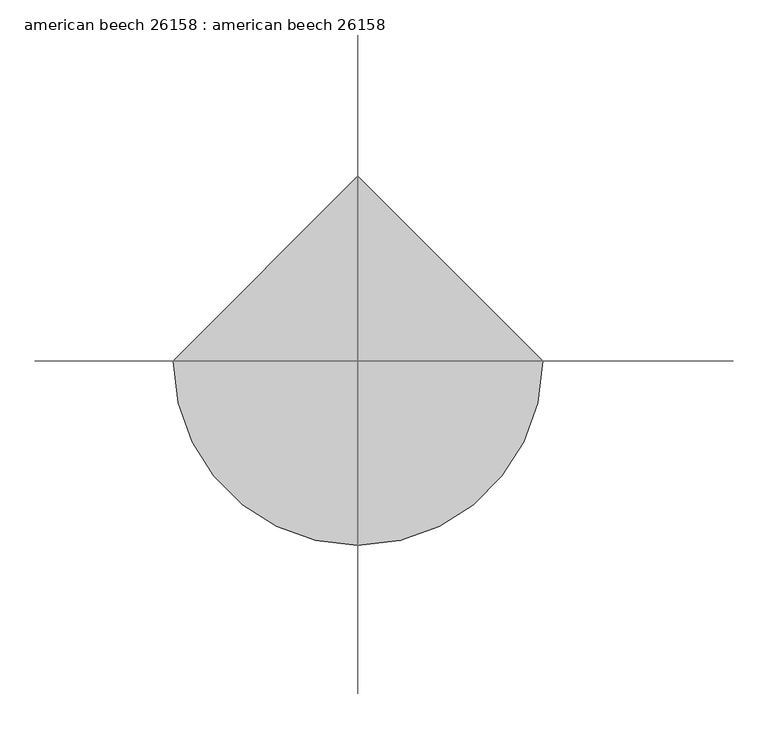
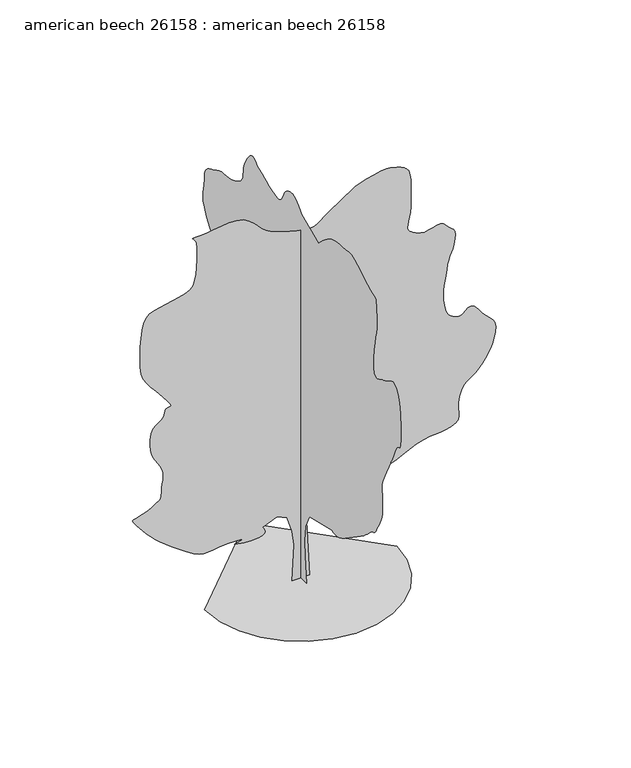
"""IFC4 building model written with IfcOpenShell, lengths in millimetres: proxy geometry, american beech 26158 : american beech 26158."""

import ifcopenshell
import ifcopenshell.guid

model = None  # the IFC model being written
_history = None  # IfcOwnerHistory: only IFC2X3 demands one
_inside = {}  # id of a spatial element -> (the spatial element, [elements in it])
_under = {}  # id of a project, library or spatial element -> (it, [spatial elements below it])
_declared = {}  # id of a project -> (the project, [libraries it declares])
_typed = {}  # id of a type object -> (the type object, [elements of that type])
_made_of = {}  # id of a material, layer set ... -> (it, [elements and type objects made of it])


def new_model(schema):
    """Start an empty IFC model of exactly this schema.

    Asked for "IFC4X3", IfcOpenShell would pick the latest addendum, in which some entities
    have other attributes; the version numbers below select the first issue.
    IFC2X3 requires an IfcOwnerHistory on every rooted entity: one is made here for all.
    """
    global model, _history
    if schema == "IFC4X3":
        model = ifcopenshell.file(schema_version=(4, 3, 0, 0))
    else:
        model = ifcopenshell.file(schema=schema)
    _inside.clear()
    _under.clear()
    _declared.clear()
    _typed.clear()
    _made_of.clear()
    _history = None
    if model.schema == "IFC2X3":
        org = make("IfcOrganization", Name="unknown")
        user = make(
            "IfcPersonAndOrganization",
            ThePerson=make("IfcPerson", FamilyName="unknown"),
            TheOrganization=org,
        )
        app = make(
            "IfcApplication",
            ApplicationDeveloper=org,
            Version="unknown",
            ApplicationFullName="unknown",
            ApplicationIdentifier="unknown",
        )
        _history = make(
            "IfcOwnerHistory",
            OwningUser=user,
            OwningApplication=app,
            ChangeAction="ADDED",
            CreationDate=0,
        )
    return model


def make(cls, **values):
    """One entity of the class cls with the attributes given. An attribute that is None is left unset."""
    return model.create_entity(
        cls, **{name: value for name, value in values.items() if value is not None}
    )


def rooted(cls, **values):
    """An entity with a GlobalId (a new one), such as an element, a storey or a relation."""
    return make(cls, GlobalId=ifcopenshell.guid.new(), OwnerHistory=_history, **values)


def si_unit(unit_type, name, prefix=None):
    """IfcSIUnit, for example si_unit("LENGTHUNIT", "METRE", prefix="MILLI")."""
    return make("IfcSIUnit", UnitType=unit_type, Prefix=prefix, Name=name)


def assignment(units):
    """IfcUnitAssignment: the units of a project."""
    return None if units is None else make("IfcUnitAssignment", Units=units)


def point(xyz):
    """IfcCartesianPoint."""
    return None if xyz is None else make("IfcCartesianPoint", Coordinates=xyz)


def direction(xyz):
    """IfcDirection."""
    return None if xyz is None else make("IfcDirection", DirectionRatios=xyz)


def frame(location, z_axis=None, x_axis=None):
    """IfcAxis2Placement3D, a coordinate frame: its origin and axes. An axis left out is left unset."""
    return make(
        "IfcAxis2Placement3D",
        Location=point(location),
        Axis=direction(z_axis),
        RefDirection=direction(x_axis),
    )


def origin():
    """The frame at (0, 0, 0) with its axes left unset."""
    return frame((0.0, 0.0, 0.0))


def place(relative_to, where):
    """IfcLocalPlacement: puts the frame where relative to a parent placement (None: the world)."""
    return make(
        "IfcLocalPlacement", PlacementRelTo=relative_to, RelativePlacement=where
    )


def context(
    kind, dimensions, precision=None, world=None, true_north=None, identifier=None
):
    """IfcGeometricRepresentationContext, for example the 3D "Model" context."""
    return make(
        "IfcGeometricRepresentationContext",
        ContextIdentifier=identifier,
        ContextType=kind,
        CoordinateSpaceDimension=dimensions,
        Precision=precision,
        WorldCoordinateSystem=world,
        TrueNorth=true_north,
    )


def project(units=None, contexts=None):
    """IfcProject with its units and contexts."""
    return rooted(
        "IfcProject",
        Name="project",
        RepresentationContexts=contexts,
        UnitsInContext=assignment(units),
    )


def spatial(cls, under=None, at=None, **own):
    """A site, building, storey or space (cls), placed at a placement, below another one or the project."""
    s = rooted(cls, ObjectPlacement=at, **own)
    if under is not None:
        _under.setdefault(under.id(), (under, []))[1].append(s)
    return s


def point_list(points):
    """IfcCartesianPointList2D or 3D."""
    cls = (
        "IfcCartesianPointList2D" if len(points[0]) == 2 else "IfcCartesianPointList3D"
    )
    return make(cls, CoordList=points)


def triangles(points, corners, closed=None, point_numbers=None):
    """IfcTriangulatedFaceSet: each triangle names its three corners, points numbered from 1."""
    return make(
        "IfcTriangulatedFaceSet",
        Coordinates=point_list(points),
        Closed=closed,
        CoordIndex=corners,
        PnIndex=point_numbers,
    )


def shape(context_of_items, identifier, shape_type, items):
    """IfcShapeRepresentation: the items that make up one representation, for example the "Body"."""
    return make(
        "IfcShapeRepresentation",
        ContextOfItems=context_of_items,
        RepresentationIdentifier=identifier,
        RepresentationType=shape_type,
        Items=items,
    )


def source(mapping_origin, context_of_items, identifier, shape_type, items):
    """IfcRepresentationMap: a shape defined once, which mapped items show again and again."""
    return make(
        "IfcRepresentationMap",
        MappingOrigin=mapping_origin,
        MappedRepresentation=shape(context_of_items, identifier, shape_type, items),
    )


def transform(
    local_origin,
    x_axis=None,
    y_axis=None,
    z_axis=None,
    scale=None,
    scale2=None,
    scale3=None,
    uniform=True,
):
    """IfcCartesianTransformationOperator3D, or its non-uniform kind. x_axis, y_axis, z_axis: its Axis1, 2, 3."""
    if uniform:
        return make(
            "IfcCartesianTransformationOperator3D",
            Axis1=direction(x_axis),
            Axis2=direction(y_axis),
            LocalOrigin=point(local_origin),
            Scale=scale,
            Axis3=direction(z_axis),
        )
    return make(
        "IfcCartesianTransformationOperator3DnonUniform",
        Axis1=direction(x_axis),
        Axis2=direction(y_axis),
        LocalOrigin=point(local_origin),
        Scale=scale,
        Axis3=direction(z_axis),
        Scale2=scale2,
        Scale3=scale3,
    )


def mapped(mapping_source, mapping_target):
    """IfcMappedItem: shows the shape of a source again, moved by a transform."""
    return make(
        "IfcMappedItem", MappingSource=mapping_source, MappingTarget=mapping_target
    )


def made_of(thing, what):
    """Note that an element or type object is made of a material, layer set ...; save() writes the relation."""
    if what is not None:
        _made_of.setdefault(what.id(), (what, []))[1].append(thing)
    return thing


def element(
    cls,
    number,
    at=None,
    inside=None,
    cuts=None,
    type_object=None,
    material=None,
    context=None,
    identifier="Body",
    shape_type=None,
    held_by="IfcProductDefinitionShape",
    body=None,
    shapes=None,
    **own,
):
    """One element of the class cls, such as IfcWall. Its Tag is "e" and its number.

    at: its placement. inside: the storey or other place that contains it. cuts: it is an
    opening in that element (IfcRelVoidsElement). A single representation is given by context,
    identifier, shape_type and body (its items); several are given by shapes. held_by: the class
    of the entity that holds the representations. save() writes the other relations.
    """
    e = rooted(cls, Tag="e%d" % number, ObjectPlacement=at, **own)
    if body is not None:
        shapes = [shape(context, identifier, shape_type, body)]
    if shapes is not None:
        e.Representation = make(held_by, Representations=shapes)
    if inside is not None:
        _inside.setdefault(inside.id(), (inside, []))[1].append(e)
    if cuts is not None:
        rooted(
            "IfcRelVoidsElement", RelatingBuildingElement=cuts, RelatedOpeningElement=e
        )
    if type_object is not None:
        _typed.setdefault(type_object.id(), (type_object, []))[1].append(e)
    return made_of(e, material)


def aggregate(whole, parts):
    """IfcRelAggregates: a whole, such as a stair, and the parts it consists of."""
    return rooted("IfcRelAggregates", RelatingObject=whole, RelatedObjects=parts)


def save(model, path):
    """Write the relations noted so far, then the file.

    IfcRelAggregates (storeys below a building ...), IfcRelContainedInSpatialStructure (elements
    in a storey), IfcRelDefinesByType, IfcRelAssociatesMaterial and IfcRelDeclares: one each for
    every whole, place, type object, material and project.
    """
    for whole, parts in _under.values():
        aggregate(whole, parts)
    for where, things in _inside.values():
        rooted(
            "IfcRelContainedInSpatialStructure",
            RelatedElements=things,
            RelatingStructure=where,
        )
    for kind, things in _typed.values():
        rooted("IfcRelDefinesByType", RelatedObjects=things, RelatingType=kind)
    for what, things in _made_of.values():
        rooted("IfcRelAssociatesMaterial", RelatedObjects=things, RelatingMaterial=what)
    for by, libraries in _declared.values():
        rooted("IfcRelDeclares", RelatingContext=by, RelatedDefinitions=libraries)
    model.write(path)


def american_beech_26158_american_beech_26158_b3c041c8(model_context):
    return source(origin(), model_context, "Body", "Tessellation", [
        triangles([(0.0009889, 136.856581, 0.0), (0.0009889, -149.8547884, 0.0), (0.0009889, -111.6264895, 420.510052), (0.0009889, -102.0697236, 659.4353302), (0.0009889, -121.1832463, 898.3606447), (0.0009889, -235.8678885, 1118.172373), (0.0009889, -818.8458761, 1261.5275036), (0.0009889, -849.9431059, 1249.7139805), (0.0009889, -883.2933231, 1240.7427258), (0.0009889, -921.1596891, 1237.4533916), (0.0009889, -965.7976622, 1242.6934788), (0.0009889, -1019.4603024, 1259.3000233), (0.0009889, -1084.4081549, 1290.1152935), (0.0009889, -1162.8992941, 1337.984174), (0.0009889, -1478.2811337, 1557.7959023), (0.0009889, -1522.8632961, 1589.1420994), (0.0009889, -1566.942437, 1618.9819931), (0.0009889, -1611.1893002, 1649.3249084), (0.0009889, -1656.2718681, 1682.1772636), (0.0009889, -1702.8579781, 1719.5406807), (0.0009889, -1751.6183739, 1763.4243393), (0.0009889, -1803.2210381, 1815.834803), (0.0009889, -1847.9404015, 1858.0191467), (0.0009889, -1878.9512993, 1877.1351311), (0.0009889, -1901.2702858, 1884.0440117), (0.0009889, -1919.9112991, 1889.616782), (0.0009889, -1939.8884228, 1904.7196392), (0.0009889, -1966.2180656, 1940.2161644), (0.0009889, -2003.916782, 2006.9774963), (0.0009889, -2044.9607883, 2083.2080177), (0.0009889, -2078.313549, 2145.2324295), (0.0009889, -2104.4754696, 2201.0692829), (0.0009889, -2123.9521877, 2258.7475937), (0.0009889, -2137.244109, 2326.2862038), (0.0009889, -2144.8488773, 2411.7141289), (0.0009889, -2147.2746014, 2523.0550072), (0.0009889, -2142.5373905, 2624.8889076), (0.0009889, -2132.7863869, 2688.2873634), (0.0009889, -2124.7040314, 2730.9338882), (0.0009889, -2124.9835201, 2770.583503), (0.0009889, -2140.3072941, 2824.9394875), (0.0009889, -2177.3659332, 2911.7568626), (0.0009889, -2242.84464, 3048.6883301), (0.0009889, -2308.7119858, 3181.9621719), (0.0009889, -2348.5011269, 3259.3812836), (0.0009889, -2371.2366577, 3301.215358), (0.0009889, -2385.9484051, 3327.6567673), (0.0009889, -2401.6632889, 3358.9496246), (0.0009889, -2427.4088104, 3415.3121727), (0.0009889, -2472.2118896, 3516.9885246), (0.0009889, -2522.8114174, 3609.6476944), (0.0009889, -2561.0332123, 3645.1568642), (0.0009889, -2588.5669968, 3652.9040657), (0.0009889, -2607.0580193, 3662.3273277), (0.0009889, -2618.2087921, 3702.8402618), (0.0009889, -2623.669796, 3803.856189), (0.0009889, -2625.117382, 3994.8390083), (0.0009889, -2615.3639076, 4210.713913), (0.0009889, -2589.2271309, 4371.4450905), (0.0009889, -2551.406765, 4483.8402649), (0.0009889, -2506.5400269, 4554.7824463), (0.0009889, -2459.3391289, 4591.1043571), (0.0009889, -2414.4802391, 4599.6895889), (0.0009889, -2376.641851, 4587.3705734), (0.0009889, -2343.8477772, 4566.9491455), (0.0009889, -2310.8862717, 4546.8576393), (0.0009889, -2277.5893215, 4527.4521378), (0.0009889, -2243.7921112, 4509.0116936), (0.0009889, -2209.3243023, 4491.9426773), (0.0009889, -2174.0232594, 4476.5250137), (0.0009889, -2137.7164639, 4463.1392029), (0.0009889, -2096.4236355, 4443.6572525), (0.0009889, -2049.6139927, 4418.4858238), (0.0009889, -2002.3013283, 4400.6805153), (0.0009889, -1959.504958, 4403.2713455), (0.0009889, -1926.2359131, 4439.313913), (0.0009889, -1907.5110386, 4521.8132378), (0.0009889, -1908.3467434, 4663.8246277), (0.0009889, -1923.6450829, 4819.4253044), (0.0009889, -1942.954224, 4940.7356323), (0.0009889, -1963.266647, 5037.9669067), (0.0009889, -1981.572361, 5121.3298416), (0.0009889, -1994.8642822, 5201.0354416), (0.0009889, -2000.1296585, 5287.2429703), (0.0009889, -1994.3614059, 5390.1634323), (0.0009889, -1986.3653824, 5488.9190323), (0.0009889, -1983.048143, 5559.911792), (0.0009889, -1978.5625156, 5609.3407516), (0.0009889, -1967.0562412, 5643.3764648), (0.0009889, -1942.6748806, 5668.2429703), (0.0009889, -1899.5709709, 5690.0869858), (0.0009889, -1831.8926891, 5715.1063889), (0.0009889, -1748.4408062, 5751.9616974), (0.0009889, -1662.820015, 5800.5261749), (0.0009889, -1576.3582867, 5853.7903656), (0.0009889, -1490.4020508, 5904.6919098), (0.0009889, -1406.2848015, 5946.2207703), (0.0009889, -1325.3426491, 5971.3924896), (0.0009889, -1248.913884, 5973.1447083), (0.0009889, -1174.2403896, 5963.3406555), (0.0009889, -1098.5636135, 5956.711409), (0.0009889, -1023.222064, 5950.5641098), (0.0009889, -949.5518515, 5942.2588028), (0.0009889, -878.8914843, 5929.1264648), (0.0009889, -812.5771454, 5908.4509827), (0.0009889, -751.9472706, 5877.5644958), (0.0009889, -697.9494038, 5841.2678741), (0.0009889, -649.9687569, 5805.9618896), (0.0009889, -607.0045916, 5771.4942261), (0.0009889, -568.0511189, 5737.7119858), (0.0009889, -532.1075644, 5704.4128555), (0.0009889, -498.1706097, 5671.4433563), (0.0009889, -465.2369368, 5638.6523346), (0.0009889, -16.056217, 5829.7871796), (0.0009889, 22.8405617, 5872.4339951), (0.0009889, 61.6537222, 5913.023378), (0.0009889, 100.2998553, 5949.3961578), (0.0009889, 138.6950317, 5979.5204819), (0.0009889, 176.7559443, 6001.2883392), (0.0009889, 214.3990318, 6012.5911377), (0.0009889, 251.5404602, 6011.3720261), (0.0009889, 287.2056524, 6002.4312927), (0.0009889, 320.3628219, 5991.305809), (0.0009889, 350.8454089, 5977.0055191), (0.0009889, 378.4856913, 5958.5397858), (0.0009889, 403.1160919, 5934.892392), (0.0009889, 424.5689612, 5905.047702), (0.0009889, 442.6817001, 5868.0144974), (0.0009889, 459.9562634, 5826.9425858), (0.0009889, 480.2407084, 5787.547316), (0.0009889, 505.3740581, 5752.6727005), (0.0009889, 537.1926464, 5725.138916), (0.0009889, 577.5380399, 5707.7911377), (0.0009889, 628.2491524, 5703.5239563), (0.0009889, 691.1650068, 5715.1063889), (0.0009889, 759.6790661, 5736.9754028), (0.0009889, 826.1890326, 5761.3593796), (0.0009889, 891.0251186, 5787.8263687), (0.0009889, 954.5251671, 5815.9694183), (0.0009889, 1017.0218611, 5845.3577408), (0.0009889, 1078.8506453, 5875.5832214), (0.0009889, 1140.3440575, 5906.2412338), (0.0009889, 1169.0715191, 5932.3524307), (0.0009889, 1198.1316639, 5955.3649796), (0.0009889, 1227.8624073, 5972.2052307), (0.0009889, 1258.5938164, 5979.7489563), (0.0009889, 1290.6664227, 5974.9230881), (0.0009889, 1324.4078224, 5954.6539764), (0.0009889, 1360.1557858, 5915.7918137), (0.0009889, 1395.1799561, 5868.217392), (0.0009889, 1426.1908539, 5822.9544571), (0.0009889, 1452.6880737, 5778.8856354), (0.0009889, 1474.1715008, 5734.7912338), (0.0009889, 1490.1379681, 5689.5538788), (0.0009889, 1500.0845993, 5641.9538773), (0.0009889, 1503.510989, 5590.8494385), (0.0009889, 1507.2168674, 5539.3380478), (0.0009889, 1519.1142517, 5491.1793594), (0.0009889, 1540.3740005, 5446.1704788), (0.0009889, 1572.1672634, 5404.1846695), (0.0009889, 1615.6596668, 5365.0428726), (0.0009889, 1672.0274471, 5328.5689362), (0.0009889, 1742.4363762, 5294.5832199), (0.0009889, 1817.5288857, 5269.1836075), (0.0009889, 1887.9378147, 5255.1373718), (0.0009889, 1954.8363476, 5247.4407486), (0.0009889, 2019.3956337, 5241.0911362), (0.0009889, 2082.7839157, 5231.0580276), (0.0009889, 2146.1721977, 5212.3382401), (0.0009889, 2210.7313385, 5179.9024292), (0.0009889, 2276.3498623, 5145.3580261), (0.0009889, 2340.1267834, 5118.8404587), (0.0009889, 2399.0573433, 5093.1356323), (0.0009889, 2450.1315514, 5061.106192), (0.0009889, 2490.3372368, 5015.5136261), (0.0009889, 2516.667025, 4949.193837), (0.0009889, 2526.1132507, 4854.9597633), (0.0009889, 2532.46577, 4758.008123), (0.0009889, 2546.5044479, 4681.9348595), (0.0009889, 2560.7285797, 4617.2411339), (0.0009889, 2567.5865913, 4554.3760757), (0.0009889, 2559.5600464, 4483.8402649), (0.0009889, 2529.1232414, 4396.0578323), (0.0009889, 2468.7702393, 4281.5543564), (0.0009889, 2394.0992157, 4166.6192207), (0.0009889, 2326.6139454, 4078.2525215), (0.0009889, 2267.6553349, 4007.9707649), (0.0009889, 2218.5596397, 3947.1884285), (0.0009889, 2180.6679119, 3887.4223091), (0.0009889, 2155.3111748, 3820.1377533), (0.0009889, 2143.8328056, 3736.8001076), (0.0009889, 2149.4334812, 3646.0204742), (0.0009889, 2171.0820145, 3561.7686401), (0.0009889, 2203.7667927, 3483.5112076), (0.0009889, 2242.4687908, 3410.790937), (0.0009889, 2282.1714546, 3343.1000107), (0.0009889, 2317.8662235, 3279.9047401), (0.0009889, 2344.5311657, 3220.7225967), (0.0009889, 2370.3577869, 3180.6921913), (0.0009889, 2402.5396889, 3164.8934464), (0.0009889, 2434.5538685, 3157.7813805), (0.0009889, 2459.8827003, 3143.8113029), (0.0009889, 2472.0037628, 3107.4638123), (0.0009889, 2464.3963783, 3033.1433487), (0.0009889, 2430.5432121, 2905.3305107), (0.0009889, 2383.9011463, 2761.3378464), (0.0009889, 2340.6017544, 2643.9136185), (0.0009889, 2298.1379219, 2545.7425758), (0.0009889, 2254.0028252, 2459.415287), (0.0009889, 2205.6894951, 2377.6095245), (0.0009889, 2150.6857304, 2292.9614937), (0.0009889, 2086.4897942, 2198.1177189), (0.0009889, 2022.098085, 2102.5196297), (0.0009889, 1968.0723129, 2019.6267242), (0.0009889, 1924.2446102, 1948.102747), (0.0009889, 1890.4447838, 1886.6067913), (0.0009889, 1866.5103436, 1833.8078339), (0.0009889, 1852.2735672, 1788.3620613), (0.0009889, 1847.564407, 1748.9361248), (0.0009889, 1851.5776794, 1721.8800728), (0.0009889, 1860.940044, 1709.2029396), (0.0009889, 1871.6386642, 1703.0459026), (0.0009889, 1879.6624477, 1695.5504299), (0.0009889, 1881.0010288, 1678.8600243), (0.0009889, 1871.6386642, 1645.1186245), (0.0009889, 1847.564407, 1586.4675533), (0.0009889, 1827.5314728, 1524.5828133), (0.0009889, 1825.3850922, 1482.2587978), (0.0009889, 1829.7590984, 1453.3104195), (0.0009889, 1829.2865982, 1431.547649), (0.0009889, 1812.5961926, 1410.7907764), (0.0009889, 1768.3214241, 1384.8497726), (0.0009889, 1685.0958355, 1347.5421661), (0.0009889, 1594.399918, 1309.4244347), (0.0009889, 1528.281134, 1282.5080544), (0.0009889, 1476.2059696, 1262.7823689), (0.0009889, 1427.6412014, 1246.2316349), (0.0009889, 1372.05317, 1228.8453415), (0.0009889, 1298.9138844, 1206.6102161), (0.0009889, 1197.6871416, 1175.5154572), (0.0009889, 1096.069289, 1145.7009253), (0.0009889, 1022.5387482, 1127.7557997), (0.0009889, 967.7331545, 1118.3400227), (0.0009889, 922.2874546, 1114.10329), (0.0009889, 876.8442255, 1111.7080873), (0.0009889, 822.0360884, 1107.806654), (0.0009889, 748.5055475, 1099.0588594), (0.0009889, 662.4935011, 1085.0990284), (0.0009889, 576.4788749, 1068.1292793), (0.0009889, 490.4667558, 1048.6551046), (0.0009889, 404.4521296, 1027.1717503), (0.0009889, 318.4400468, 1004.1847086), (0.0009889, 232.4266923, 980.1943851), (0.0009889, 146.4133378, 955.7037289), (136.1842383, 0.0003154, 0.014068), (-131.4120823, 0.0003154, 0.014068), (-102.7410489, 0.0002819, 563.8778998), (-131.4120823, 0.0002692, 793.2477293), (-207.8684348, 0.0002549, 1032.1729712), (-360.7819027, 0.0002501, 1108.6296415), (-580.5936673, 0.0002549, 1013.0594576), (-562.704425, 0.0002564, 988.5662579), (-548.0765751, 0.000258, 964.5784779), (-539.9688578, 0.0002596, 941.5914362), (-541.6401947, 0.0002612, 920.1080818), (-556.3518694, 0.0002628, 900.6313637), (-587.3627672, 0.0002628, 883.6641581), (-637.9342443, 0.0002644, 869.704327), (-697.421093, 0.0002644, 860.4815615), (-753.4001616, 0.0002644, 856.775683), (-806.4506298, 0.0002644, 857.667271), (-857.1617786, 0.0002644, 862.2366869), (-906.117802, 0.0002644, 869.5645826), (-953.9028214, 0.0002628, 878.731465), (-1001.1011759, 0.0002628, 888.8178406), (-953.2881786, 0.0002628, 900.9945683), (-913.501581, 0.0002612, 912.5008427), (-889.7601522, 0.0002612, 922.6710068), (-890.0954515, 0.0002596, 930.8345346), (-922.5287189, 0.0002596, 936.3235165), (-995.0838833, 0.0002596, 938.4698244), (-1115.7848007, 0.0002596, 936.6028599), (-1242.9524746, 0.0002612, 927.8271601), (-1337.3542706, 0.0002612, 914.3677345), (-1410.6891838, 0.0002612, 903.2500992), (-1474.6617325, 0.0002612, 901.4949738), (-1540.9759987, 0.0002612, 916.12286), (-1621.3340298, 0.0002596, 954.1568756), (-1727.4351116, 0.0002549, 1022.614979), (-1845.0726986, 0.0002501, 1105.8432564), (-1952.34711, 0.0002453, 1184.0549795), (-2049.4209812, 0.0002405, 1258.0858532), (-2136.46436, 0.0002373, 1328.7765965), (-2213.6472942, 0.0002326, 1396.9554291), (-2281.1300938, 0.0002278, 1463.4653229), (-2339.0852772, 0.0002246, 1529.1396572), (-2391.8031349, 0.0002214, 1592.6651402), (-2441.3431343, 0.0002166, 1651.1791557), (-2484.5309052, 0.0002134, 1703.170459), (-2518.1884438, 0.0002118, 1747.1378334), (-2539.1409439, 0.0002103, 1781.577737), (-2544.218541, 0.0002087, 1804.9838665), (-2530.2254997, 0.0002071, 1815.8500637), (-2498.742247, 0.0002071, 1822.7308937), (-2456.2227493, 0.0002071, 1834.628278), (-2406.8475655, 0.0002055, 1850.7065117), (-2354.8003063, 0.0002039, 1870.1272739), (-2304.2568798, 0.0002023, 1892.0551506), (-2259.3978447, 0.0002023, 1915.6542915), (-2224.401725, 0.0002007, 1940.091608), (-2196.9849392, 0.0001991, 1958.6464348), (-2172.4078056, 0.0001991, 1969.1798035), (-2151.1759621, 0.0001975, 1977.7066086), (-2133.7896687, 0.0001975, 1990.2439247), (-2120.7518017, 0.0001959, 2012.8144947), (-2112.5602959, 0.0001927, 2051.4326317), (-2109.7180275, 0.0001895, 2112.118317), (-2105.7607109, 0.0001864, 2181.0514641), (-2096.7894562, 0.0001816, 2242.2935108), (-2087.1476028, 0.0001784, 2298.6891964), (-2081.1861935, 0.0001752, 2353.0781731), (-2083.2487129, 0.000172, 2408.3028545), (-2097.6809715, 0.0001688, 2467.2028931), (-2128.8315411, 0.0001641, 2532.6259346), (-2168.3971493, 0.0001609, 2596.7202782), (-2204.2849297, 0.0001577, 2653.2860115), (-2235.1560104, 0.0001545, 2707.6675758), (-2259.6771881, 0.0001513, 2765.2239464), (-2276.5047947, 0.0001465, 2831.3149704), (-2284.3076614, 0.0001418, 2911.2740433), (-2281.7447365, 0.000137, 3010.4865921), (-2264.5514545, 0.0001306, 3102.7902603), (-2233.1494469, 0.0001274, 3164.9948936), (-2193.2231049, 0.0001242, 3206.8286774), (-2150.4520237, 0.0001226, 3237.9439293), (-2110.525827, 0.0001211, 3268.0682533), (-2079.123674, 0.0001179, 3306.8795471), (-2061.9330082, 0.0001147, 3364.0804161), (-2043.9599773, 0.0001131, 3413.0262657), (-2014.1200836, 0.0001115, 3431.3396828), (-1983.9422745, 0.0001115, 3435.3019409), (-1964.9684326, 0.0001099, 3441.0931572), (-1968.7301216, 0.0001099, 3464.9437363), (-2006.7641373, 0.0001051, 3523.0843735), (-2090.6020432, 9.88e-05, 3631.6948952), (-2191.4121689, 9.24e-05, 3753.7165169), (-2273.3296978, 8.6e-05, 3849.6778107), (-2337.3582024, 8.12e-05, 3932.1009773), (-2384.5031445, 7.65e-05, 4013.5079269), (-2415.7654804, 7.17e-05, 4106.47202), (-2432.1484921, 6.37e-05, 4223.4898773), (-2434.6554611, 5.42e-05, 4377.1345688), (-2429.5297565, 4.46e-05, 4541.5998207), (-2420.5585018, 3.66e-05, 4683.0016548), (-2405.0643894, 3.03e-05, 4801.6705742), (-2380.3781055, 2.39e-05, 4897.9365005), (-2343.822488, 1.91e-05, 4972.1558075), (-2292.720084, 1.59e-05, 5024.6066757), (-2224.401725, 1.43e-05, 5055.6710587), (-2138.4149677, 1.27e-05, 5074.7972168), (-2040.8941761, 1.27e-05, 5092.7292618), (-1939.0274288, 1.11e-05, 5111.8554199), (-1840.0028046, 9.6e-06, 5134.487178), (-1751.0088181, 8e-06, 5162.9604401), (-1679.2334026, 6.4e-06, 5199.612854), (-1631.8649277, 3.2e-06, 5246.8314835), (-1604.1128426, -1.6e-06, 5316.4272354), (-1585.3905842, -6.4e-06, 5411.6010773), (-1574.1890877, -1.27e-05, 5521.6594757), (-1569.0075726, -2.07e-05, 5635.9088974), (-1568.336974, -2.71e-05, 5743.6302292), (-1570.6788368, -3.19e-05, 5834.1305191), (-1574.524387, -3.5e-05, 5896.690654), (-1585.918895, -3.82e-05, 5936.1626633), (-1606.0102558, -3.98e-05, 5965.4230865), (-1625.9315689, -4.14e-05, 5985.9718323), (-1636.825526, -4.14e-05, 5999.3576431), (-1629.8329296, -4.3e-05, 6007.0286865), (-1596.0890591, -4.3e-05, 6010.559285), (-1526.7393677, -4.3e-05, 6011.3976059), (-1428.7715103, -4.3e-05, 6017.8233765), (-1318.7690678, -4.46e-05, 6032.4538788), (-1202.2439129, -4.46e-05, 6048.2529144), (-1084.7180197, -4.46e-05, 6058.184285), (-971.7057318, -4.46e-05, 6055.263533), (-868.7238636, -4.46e-05, 6032.4538788), (-781.2893749, -4.14e-05, 5982.7208679), (-714.8937183, -3.66e-05, 5922.6245361), (-665.5465851, -3.34e-05, 5871.6974121), (-624.5610781, -3.19e-05, 5827.4756927), (-583.2403444, -2.87e-05, 5787.445578), (-532.8924365, -2.71e-05, 5749.0915237), (-464.8228995, -2.39e-05, 5709.8735687), (-370.3373878, -2.23e-05, 5667.3284912), (-260.8632923, -1.91e-05, 5627.3745346), (-155.7366604, -1.75e-05, 5596.9449966), (-58.1322665, -1.59e-05, 5575.0504028), (28.7726351, -1.59e-05, 5560.6739548), (101.8020074, -1.59e-05, 5552.8255966), (157.7788323, -1.43e-05, 5550.4629501), (193.5270681, -1.59e-05, 5552.6477005), (219.2725352, -1.59e-05, 5560.6233765), (247.3583572, -1.59e-05, 5575.4311935), (277.7847885, -1.75e-05, 5595.7770447), (310.5508118, -1.91e-05, 5620.2877579), (345.6587342, -2.07e-05, 5647.6692261), (383.1059761, -2.23e-05, 5676.5232788), (422.8950809, -2.39e-05, 5705.555809), (805.1781057, -3.98e-05, 5963.5947098), (830.3647951, -3.98e-05, 5972.992392), (896.679134, -4.14e-05, 5996.5892075), (990.2426817, -4.3e-05, 6027.5518524), (1097.1817938, -4.62e-05, 6058.9970261), (1203.6180296, -4.62e-05, 6084.1175858), (1295.67789, -4.78e-05, 6096.0046509), (1359.4853325, -4.78e-05, 6087.8516602), (1407.4912685, -4.62e-05, 6070.6556168), (1459.1777939, -4.46e-05, 6056.8128571), (1511.1996185, -4.46e-05, 6041.4457718), (1560.2089817, -4.3e-05, 6019.7540726), (1602.8682964, -4.14e-05, 5986.835733), (1635.8299473, -3.82e-05, 5937.8898834), (1655.7537312, -3.34e-05, 5868.0394958), (1665.3091072, -2.87e-05, 5789.7820633), (1670.1859898, -2.55e-05, 5717.2399796), (1671.5500053, -2.07e-05, 5647.8471222), (1670.5746288, -1.75e-05, 5579.1396881), (1668.4282482, -1.27e-05, 5508.6038773), (1666.2844837, -8e-06, 5433.699147), (1665.3091072, -3.2e-06, 5351.9622757), (1660.2367424, 1.6e-06, 5270.5806152), (1648.1463467, 6.4e-06, 5198.4187408), (1633.7114719, 9.6e-06, 5135.2743393), (1621.6186054, 1.27e-05, 5081.0200928), (1616.5487114, 1.59e-05, 5035.4269455), (1623.1807194, 1.75e-05, 4998.368161), (1646.1955936, 1.91e-05, 4969.6664246), (1678.4054008, 2.07e-05, 4946.8317719), (1709.6119263, 2.23e-05, 4927.324823), (1739.9826015, 2.23e-05, 4910.992099), (1769.6829689, 2.39e-05, 4897.6824463), (1798.8852562, 2.39e-05, 4887.1923889), (1827.7499187, 2.55e-05, 4879.3946091), (1856.4493298, 2.55e-05, 4874.0862122), (1893.0609032, 2.55e-05, 4877.1087021), (1942.2125542, 2.39e-05, 4889.9864044), (1998.8851124, 2.39e-05, 4906.1918106), (2058.0671104, 2.23e-05, 4919.2474091), (2114.7396687, 2.23e-05, 4922.5745316), (2163.8911743, 2.39e-05, 4909.6968292), (2200.5028931, 2.55e-05, 4874.0862122), (2230.4850746, 2.71e-05, 4834.208123), (2261.3003448, 2.87e-05, 4807.6649757), (2290.2766285, 3.03e-05, 4786.8368866), (2314.7419956, 3.19e-05, 4763.9769447), (2332.0165226, 3.34e-05, 4731.4396866), (2339.4282795, 3.66e-05, 4681.5031998), (2334.3025749, 4.14e-05, 4606.4970222), (2319.8956055, 4.62e-05, 4526.9440292), (2302.1485783, 4.94e-05, 4463.951944), (2282.3925167, 5.26e-05, 4410.6627548), (2261.9683273, 5.57e-05, 4360.1928703), (2242.2147366, 5.89e-05, 4305.7098587), (2224.4652386, 6.37e-05, 4240.3809975), (2210.0608852, 6.85e-05, 4157.3229858), (2196.9087811, 7.33e-05, 4068.4481781), (2183.2562714, 7.8e-05, 3988.0827347), (2170.9397266, 8.28e-05, 3913.0762665), (2161.8007496, 8.76e-05, 3840.2289688), (2157.6783268, 9.08e-05, 3766.3913246), (2160.4088287, 9.56e-05, 3688.3876556), (2171.831242, 0.0001003, 3603.0181572), (2189.9719952, 0.0001051, 3525.0147789), (2211.6203831, 0.0001083, 3468.2711494), (2236.7791672, 0.0001115, 3428.240744), (2265.4506729, 0.0001131, 3400.402327), (2297.6324295, 0.0001147, 3380.2602425), (2333.3271984, 0.0001147, 3363.2673843), (2372.5296021, 0.0001163, 3344.9795471), (2412.5675652, 0.0001163, 3342.4901642), (2451.7724396, 0.0001147, 3366.0869797), (2491.642971, 0.0001131, 3400.8848557), (2533.6901138, 0.0001115, 3432.0253967), (2579.4227875, 0.0001099, 3444.5728867), (2630.3246223, 0.0001115, 3423.7195084), (2687.906282, 0.0001163, 3354.5298363), (2749.8568611, 0.0001211, 3269.9730789), (2810.1313797, 0.0001242, 3206.9557045), (2864.6905495, 0.0001274, 3156.6637161), (2909.5976921, 0.0001306, 3110.2325386), (2940.7635223, 0.0001338, 3058.7720169), (2954.2254913, 0.000137, 2993.4178665), (2945.9451828, 0.0001434, 2905.3557999), (2924.1520363, 0.0001481, 2810.6139084), (2899.209082, 0.0001529, 2729.079641), (2870.2277115, 0.0001577, 2657.6040619), (2836.3948929, 0.0001609, 2592.9612053), (2796.8723053, 0.0001641, 2531.9858574), (2750.8474983, 0.0001688, 2471.5235596), (2697.4568619, 0.000172, 2408.3842449), (2642.4404526, 0.0001752, 2354.2186558), (2591.9196991, 0.0001784, 2316.7713776), (2545.7425758, 0.00018, 2287.0127289), (2503.7637428, 0.0001816, 2255.9181152), (2465.7858284, 0.0001832, 2214.4575645), (2431.6531734, 0.000188, 2153.606773), (2401.2011078, 0.0001927, 2064.3332977), (2384.7901909, 0.0001991, 1965.7532684), (2385.7654221, 0.0002039, 1881.8849865), (2393.4261463, 0.0002071, 1811.0570423), (2397.0760689, 0.0002118, 1751.5981716), (2386.0143894, 0.000215, 1701.8343487), (2349.5424877, 0.0002166, 1660.0945999), (2276.9594181, 0.0002182, 1624.7096958), (2189.7484623, 0.0002198, 1601.1638947), (2111.7322941, 0.0002214, 1590.8261536), (2035.7202187, 0.0002214, 1585.8401207), (1954.5264828, 0.0002214, 1578.3445026), (1860.9630077, 0.000223, 1560.4858543), (1747.8389534, 0.0002246, 1524.4025917), (1607.9660957, 0.0002294, 1462.2385082), (1455.667543, 0.0002326, 1390.7425816), (1311.7282185, 0.0002357, 1331.4512878), (1178.6524023, 0.0002389, 1283.6941738), (1058.9547667, 0.0002421, 1246.8031116), (955.1372663, 0.0002437, 1220.1102642), (869.7094139, 0.0002437, 1202.9449602), (805.1781057, 0.0002453, 1194.641688), (403.7815673, 0.0002453, 1185.0862392), (107.513205, 0.0002485, 1137.3011473), (88.3996914, 0.0002628, 879.2597757), (-1453.7574852, 0.0, 0.0120292), (-1415.3246567, -333.1060121, 0.0120292), (-1305.8708725, -639.0085974, 0.0120292), (-1134.1566444, -908.9473532, 0.0120292), (-908.9473532, -1134.1566444, 0.0120292), (-639.0085974, -1305.8708725, 0.0120292), (-333.1060121, -1415.3246567, 0.0120292), (6.35e-05, -1453.7574852, 0.0120292), (333.1060121, -1415.3246567, 0.0120292), (639.0085974, -1305.8708725, 0.0120292), (908.9473532, -1134.1566444, 0.0120292), (1134.1566444, -908.9473532, 0.0120292), (1305.8708725, -639.0085974, 0.0120292), (1415.3246567, -333.1060121, 0.0120292), (1453.7574852, 0.0001274, 0.0120292), (-0.0001906, 1453.7574852, 0.0120292)], [[1, 2, 3], [254, 1, 3], [254, 3, 4], [254, 4, 5], [254, 5, 6], [53, 54, 55], [52, 53, 55], [201, 202, 203], [201, 203, 204], [200, 201, 204], [222, 223, 224], [52, 55, 56], [200, 204, 205], [199, 200, 205], [253, 254, 6], [221, 222, 224], [221, 224, 225], [229, 230, 231], [229, 231, 232], [228, 229, 232], [228, 232, 233], [227, 228, 233], [252, 253, 6], [221, 225, 226], [220, 221, 226], [199, 205, 206], [198, 199, 206], [62, 63, 64], [61, 62, 64], [61, 64, 65], [60, 61, 65], [60, 65, 66], [59, 60, 66], [59, 66, 67], [59, 67, 68], [58, 59, 68], [58, 68, 69], [58, 69, 70], [57, 58, 70], [57, 70, 71], [57, 71, 72], [57, 72, 73], [57, 73, 74], [56, 57, 74], [52, 56, 74], [51, 52, 74], [50, 51, 74], [50, 74, 75], [49, 50, 75], [48, 49, 75], [47, 48, 75], [46, 47, 75], [45, 46, 75], [44, 45, 75], [43, 44, 75], [42, 43, 75], [42, 75, 76], [41, 42, 76], [227, 233, 234], [226, 227, 234], [220, 226, 234], [219, 220, 234], [219, 234, 235], [219, 235, 236], [219, 236, 237], [218, 219, 237], [218, 237, 238], [218, 238, 239], [218, 239, 240], [217, 218, 240], [217, 240, 241], [217, 241, 242], [217, 242, 243], [217, 243, 244], [217, 244, 245], [217, 245, 246], [216, 217, 246], [216, 246, 247], [215, 216, 247], [215, 247, 248], [251, 252, 6], [88, 89, 90], [88, 90, 91], [87, 88, 91], [87, 91, 92], [86, 87, 92], [86, 92, 93], [85, 86, 93], [84, 85, 93], [84, 93, 94], [83, 84, 94], [82, 83, 94], [81, 82, 94], [81, 94, 95], [80, 81, 95], [80, 95, 96], [80, 96, 97], [80, 97, 98], [80, 98, 99], [80, 99, 100], [80, 100, 101], [80, 101, 102], [80, 102, 103], [80, 103, 104], [80, 104, 105], [80, 105, 106], [80, 106, 107], [80, 107, 108], [80, 108, 109], [80, 109, 110], [80, 110, 111], [80, 111, 112], [79, 80, 112], [79, 112, 113], [78, 79, 113], [77, 78, 113], [76, 77, 113], [41, 76, 113], [40, 41, 113], [40, 113, 114], [39, 40, 114], [198, 206, 207], [197, 198, 207], [196, 197, 207], [196, 207, 208], [195, 196, 208], [195, 208, 209], [195, 209, 210], [195, 210, 211], [194, 195, 211], [194, 211, 212], [194, 212, 213], [193, 194, 213], [193, 213, 214], [214, 215, 248], [193, 214, 248], [193, 248, 249], [192, 193, 249], [192, 249, 250], [192, 250, 251], [192, 251, 6], [192, 6, 7], [191, 192, 7], [190, 191, 7], [189, 190, 7], [38, 39, 114], [37, 38, 114], [36, 37, 114], [35, 36, 114], [34, 35, 114], [33, 34, 114], [32, 33, 114], [31, 32, 114], [30, 31, 114], [29, 30, 114], [28, 29, 114], [27, 28, 114], [26, 27, 114], [25, 26, 114], [24, 25, 114], [23, 24, 114], [22, 23, 114], [21, 22, 114], [20, 21, 114], [19, 20, 114], [18, 19, 114], [17, 18, 114], [16, 17, 114], [15, 16, 114], [14, 15, 114], [13, 14, 114], [12, 13, 114], [11, 12, 114], [10, 11, 114], [9, 10, 114], [8, 9, 114], [7, 8, 114], [189, 7, 114], [188, 189, 114], [188, 114, 115], [188, 115, 116], [188, 116, 117], [188, 117, 118], [188, 118, 119], [188, 119, 120], [188, 120, 121], [146, 147, 148], [145, 146, 148], [144, 145, 148], [144, 148, 149], [143, 144, 149], [143, 149, 150], [142, 143, 150], [142, 150, 151], [142, 151, 152], [141, 142, 152], [141, 152, 153], [141, 153, 154], [141, 154, 155], [141, 155, 156], [140, 141, 156], [140, 156, 157], [139, 140, 157], [138, 139, 157], [138, 157, 158], [137, 138, 158], [137, 158, 159], [136, 137, 159], [135, 136, 159], [135, 159, 160], [134, 135, 160], [134, 160, 161], [174, 175, 176], [173, 174, 176], [173, 176, 177], [172, 173, 177], [171, 172, 177], [171, 177, 178], [170, 171, 178], [170, 178, 179], [169, 170, 179], [168, 169, 179], [167, 168, 179], [166, 167, 179], [165, 166, 179], [165, 179, 180], [165, 180, 181], [165, 181, 182], [165, 182, 183], [165, 183, 184], [165, 184, 185], [165, 185, 186], [165, 186, 187], [164, 165, 187], [164, 187, 188], [163, 164, 188], [162, 163, 188], [161, 162, 188], [134, 161, 188], [133, 134, 188], [132, 133, 188], [125, 126, 127], [124, 125, 127], [124, 127, 128], [123, 124, 128], [122, 123, 128], [121, 122, 128], [121, 128, 129], [121, 129, 130], [121, 130, 131], [188, 121, 131], [132, 188, 131], [274, 275, 276], [531, 255, 256], [531, 256, 257], [531, 257, 258], [531, 258, 259], [530, 531, 259], [376, 377, 378], [376, 378, 379], [375, 376, 379], [273, 274, 276], [273, 276, 277], [375, 379, 380], [374, 375, 380], [273, 277, 278], [272, 273, 278], [301, 302, 303], [301, 303, 304], [300, 301, 304], [300, 304, 305], [299, 300, 305], [299, 305, 306], [298, 299, 306], [298, 306, 307], [297, 298, 307], [297, 307, 308], [271, 272, 278], [296, 297, 308], [296, 308, 309], [373, 374, 380], [373, 380, 381], [372, 373, 381], [295, 296, 309], [295, 309, 310], [294, 295, 310], [294, 310, 311], [294, 311, 312], [294, 312, 313], [293, 294, 313], [293, 313, 314], [292, 293, 314], [271, 278, 279], [291, 292, 314], [530, 259, 260], [372, 381, 382], [371, 372, 382], [291, 314, 315], [290, 291, 315], [371, 382, 383], [370, 371, 383], [370, 383, 384], [369, 370, 384], [369, 384, 385], [369, 385, 386], [369, 386, 387], [369, 387, 388], [369, 388, 389], [369, 389, 390], [368, 369, 390], [368, 390, 391], [367, 368, 391], [367, 391, 392], [367, 392, 393], [366, 367, 393], [366, 393, 394], [270, 271, 279], [366, 394, 395], [338, 339, 340], [338, 340, 341], [289, 290, 315], [483, 484, 485], [483, 485, 486], [482, 483, 486], [481, 482, 486], [481, 486, 487], [480, 481, 487], [288, 289, 315], [287, 288, 315], [286, 287, 315], [285, 286, 315], [284, 285, 315], [283, 284, 315], [282, 283, 315], [282, 315, 316], [281, 282, 316], [281, 316, 317], [281, 317, 318], [281, 318, 319], [281, 319, 320], [280, 281, 320], [280, 320, 321], [279, 280, 321], [279, 321, 322], [480, 487, 488], [264, 265, 266], [263, 264, 266], [263, 266, 267], [262, 263, 267], [262, 267, 268], [261, 262, 268], [261, 268, 269], [261, 269, 270], [261, 270, 279], [261, 279, 322], [260, 261, 322], [530, 260, 322], [530, 322, 323], [529, 530, 323], [529, 323, 324], [366, 395, 396], [365, 366, 396], [337, 338, 341], [337, 341, 342], [529, 324, 325], [528, 529, 325], [527, 528, 325], [526, 527, 325], [525, 526, 325], [524, 525, 325], [523, 524, 325], [522, 523, 325], [521, 522, 325], [521, 325, 326], [521, 326, 327], [521, 327, 328], [521, 328, 329], [521, 329, 330], [521, 330, 331], [521, 331, 332], [521, 332, 333], [521, 333, 334], [521, 334, 335], [521, 335, 336], [521, 336, 337], [521, 337, 342], [520, 521, 342], [520, 342, 343], [519, 520, 343], [518, 519, 343], [518, 343, 344], [517, 518, 344], [449, 450, 451], [448, 449, 451], [448, 451, 452], [447, 448, 452], [446, 447, 452], [446, 452, 453], [516, 517, 344], [515, 516, 344], [514, 515, 344], [513, 514, 344], [512, 513, 344], [511, 512, 344], [510, 511, 344], [509, 510, 344], [508, 509, 344], [507, 508, 344], [506, 507, 344], [505, 506, 344], [504, 505, 344], [503, 504, 344], [502, 503, 344], [501, 502, 344], [500, 501, 344], [499, 500, 344], [498, 499, 344], [497, 498, 344], [496, 497, 344], [495, 496, 344], [494, 495, 344], [493, 494, 344], [492, 493, 344], [491, 492, 344], [490, 491, 344], [489, 490, 344], [488, 489, 344], [480, 488, 344], [479, 480, 344], [478, 479, 344], [477, 478, 344], [476, 477, 344], [475, 476, 344], [474, 475, 344], [473, 474, 344], [472, 473, 344], [471, 472, 344], [470, 471, 344], [469, 470, 344], [468, 469, 344], [467, 468, 344], [466, 467, 344], [465, 466, 344], [464, 465, 344], [463, 464, 344], [463, 344, 345], [462, 463, 345], [462, 345, 346], [461, 462, 346], [460, 461, 346], [459, 460, 346], [458, 459, 346], [457, 458, 346], [456, 457, 346], [455, 456, 346], [454, 455, 346], [453, 454, 346], [446, 453, 346], [445, 446, 346], [444, 445, 346], [443, 444, 346], [442, 443, 346], [441, 442, 346], [440, 441, 346], [439, 440, 346], [438, 439, 346], [437, 438, 346], [436, 437, 346], [435, 436, 346], [435, 346, 347], [435, 347, 348], [435, 348, 349], [435, 349, 350], [435, 350, 351], [435, 351, 352], [435, 352, 353], [435, 353, 354], [435, 354, 355], [435, 355, 356], [435, 356, 357], [435, 357, 358], [435, 358, 359], [435, 359, 360], [435, 360, 361], [435, 361, 362], [435, 362, 363], [435, 363, 364], [435, 364, 365], [435, 365, 396], [435, 396, 397], [435, 397, 398], [435, 398, 399], [435, 399, 400], [435, 400, 401], [435, 401, 402], [435, 402, 403], [435, 403, 404], [435, 404, 405], [435, 405, 406], [435, 406, 407], [435, 407, 408], [435, 408, 409], [434, 435, 409], [433, 434, 409], [432, 433, 409], [431, 432, 409], [430, 431, 409], [429, 430, 409], [429, 409, 410], [429, 410, 411], [429, 411, 412], [428, 429, 412], [428, 412, 413], [427, 428, 413], [426, 427, 413], [426, 413, 414], [425, 426, 414], [425, 414, 415], [425, 415, 416], [425, 416, 417], [424, 425, 417], [424, 417, 418], [423, 424, 418], [423, 418, 419], [422, 423, 419], [422, 419, 420], [421, 422, 420], [546, 547, 532], [545, 546, 532], [545, 532, 533], [544, 545, 533], [544, 533, 534], [544, 534, 535], [543, 544, 535], [542, 543, 535], [542, 535, 536], [542, 536, 537], [542, 537, 538], [542, 538, 539], [542, 539, 540], [542, 540, 541]], closed=False),
    ])


if __name__ == "__main__":
    model = new_model("IFC4")
    model_context = context("Model", 3, world=origin())
    ifc_project = project(units=[si_unit("LENGTHUNIT", "METRE", prefix="MILLI")], contexts=[model_context])
    site = spatial("IfcSite", under=ifc_project)
    building = spatial("IfcBuilding", under=site)
    placement = place(None, origin())
    american_beech_26158_american_beech_26158_shape = american_beech_26158_american_beech_26158_b3c041c8(model_context)
    element("IfcBuildingElementProxy", 1, Name="american beech 26158 : american beech 26158", ObjectType="american beech 26158 : american beech 26158", at=placement, inside=building, context=model_context, shape_type="MappedRepresentation", body=[
        mapped(american_beech_26158_american_beech_26158_shape, transform((0.0, 0.0, 0.0), x_axis=(1.0, 0.0, 0.0), y_axis=(0.0, 1.0, 0.0), z_axis=(0.0, 0.0, 1.0))),
    ])
    save(model, "model.ifc")

# Revit data of these elements
# Type "american beech 26158 : american beech 26158"
#   built-in parameter 1005195 = "RPC-16-G1GQ-43Q0-7NP3-0000-ST1L-LVER-AU"
#   Height = 0
